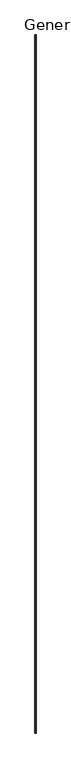
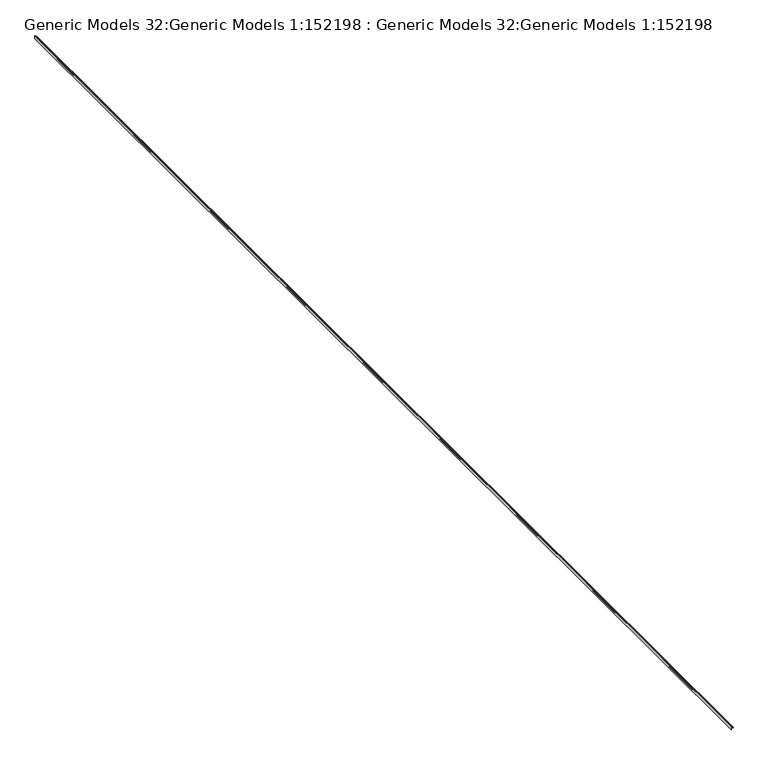
"""IFC4 building model written with IfcOpenShell, lengths in millimetres: proxy geometry, Generic Models 32:Generic Models 1:152198 : Generic Models 32:Generic Models 1:152198."""

from ifc_helpers import new_model, si_unit, frame, origin, place, context, project, spatial, polyline, outline, extrude, source, transform, mapped, element, save


def generic_models_32_generic_models_1_152198_generic_models_32_1466957d(model_context):
    return source(origin(), model_context, "Body", "SweptSolid", [
        extrude(outline(polyline([(3411.22, -9296.521787), (3371.85, -9296.521787), (3371.85, -9295.251787), (3390.9, -9295.251787), (3390.9, -9274.296787), (3395.6498, -9274.296787), (3395.6498, -9275.566787), (3392.17, -9275.566787), (3392.17, -9295.251787), (3411.22, -9295.251787), (3411.22, -9296.521787)])), frame((0.0, -6877.9974793, 0.0), z_axis=(0.0, 1.0, 0.0), x_axis=(0.0, 0.0, 1.0)), (0.0, 0.0, 1.0), 14122.4),
    ])


if __name__ == "__main__":
    model = new_model("IFC4")
    model_context = context("Model", 3, world=origin())
    ifc_project = project(units=[si_unit("LENGTHUNIT", "METRE", prefix="MILLI")], contexts=[model_context])
    site = spatial("IfcSite", under=ifc_project)
    building = spatial("IfcBuilding", under=site)
    placement = place(None, origin())
    generic_models_32_generic_models_1_152198_generic_models_32_shape = generic_models_32_generic_models_1_152198_generic_models_32_1466957d(model_context)
    element("IfcBuildingElementProxy", 1, Name="Generic Models 32:Generic Models 1:152198 : Generic Models 32:Generic Models 1:152198", ObjectType="Generic Models 32:Generic Models 1:152198 : Generic Models 32:Generic Models 1:152198", at=placement, inside=building, context=model_context, shape_type="MappedRepresentation", body=[
        mapped(generic_models_32_generic_models_1_152198_generic_models_32_shape, transform((0.0, 0.0, 0.0), x_axis=(1.0, 0.0, 0.0), y_axis=(0.0, 1.0, 0.0), z_axis=(0.0, 0.0, 1.0))),
    ])
    save(model, "model.ifc")

# Revit data of these elements
# Type "Generic Models 32:Generic Models 1:152198 : Generic Models 32:Generic Models 1:152198"
#   NameOverride = "Generic Models 32:Generic Models 1:152198"
#   ObjectTypeOverride = "Generic Models 32:Generic Models 1"
#   Reference = "Generic Models 1"
#   Category = "Generic Models"
#   Tag = "152198"
# Element 1 (IfcBuildingElementProxy, "Generic Models 32:Generic Models 1:152198 : Generic Models 32:Generic Models 1:152198")
#   Materials on its faces: "_ 16 GA. COPPER VENTED T REVEAL BEAD (CONT. AROUND PERIMETER OF BEAM) 2987"
# Materials
#   "_ 16 GA. COPPER VENTED T REVEAL BEAD (CONT. AROUND PERIMETER OF BEAM) 2987": class "Unassigned", colour RGB 253 192 103, transparency 0
